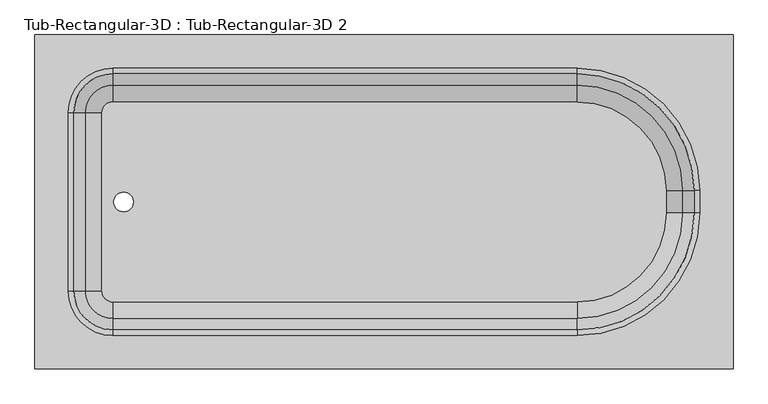
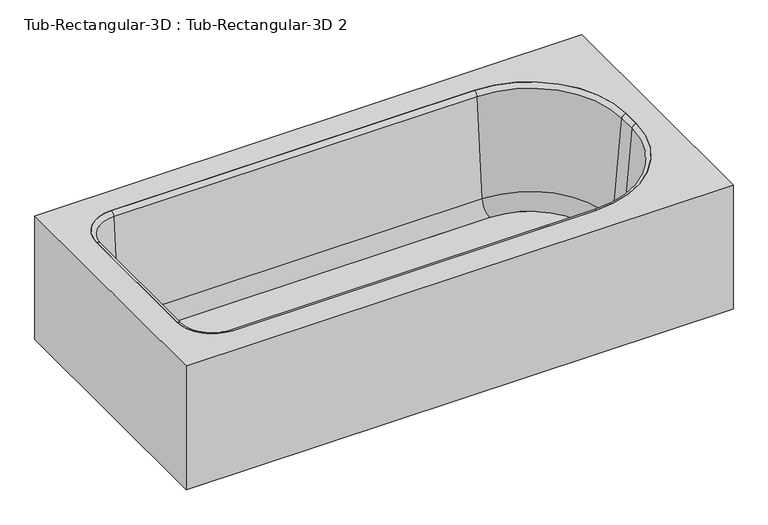
"""IFC4 building model written with IfcOpenShell, lengths in millimetres: flow terminal geometry, Tub-Rectangular-3D : Tub-Rectangular-3D 2."""

from ifc_helpers import new_model, si_unit, point, frame, frame_2d, origin, place, context, project, spatial, polyline, circle_curve, ellipse_curve, trimmed, segment, composite_curve, outline, extrude, source, transform, mapped, element, save
from ifc_brep_helpers import plane_surface, cylinder_surface, revolved_surface, advanced_brep


def tub_rectangular_3d_tub_rectangular_3d_2_a7e7f6cb(model_context):
    return source(origin(), model_context, "Body", "SolidModel", [
        advanced_brep(
        [(480.0720313, 822.325, 381.0), (-1110.6029687, 822.325, 381.0), (-1110.6029687, 60.325, 381.0), (480.0720313, 60.325, 381.0), (-932.8029687, 746.125, 381.0), (124.4720313, 746.125, 381.0), (403.8720313, 466.725, 381.0), (403.8720313, 415.925, 381.0), (124.4720313, 136.525, 381.0), (-932.8029687, 136.525, 381.0), (-1034.4029687, 238.125, 381.0), (-1034.4029687, 644.525, 381.0), (461.0220313, 803.275, 361.95), (461.0220313, 79.375, 361.95), (-1091.5529687, 79.375, 361.95), (-1091.5529687, 803.275, 361.95), (-932.8029687, 746.125, 361.95), (-1034.4029687, 644.525, 361.95), (-1034.4029687, 238.125, 361.95), (-932.8029687, 136.525, 361.95), (124.4720313, 136.525, 361.95), (403.8720313, 415.925, 361.95), (403.8720313, 466.725, 361.95), (124.4720313, 746.125, 361.95), (480.0720313, 822.325, 0.0), (-1110.6029687, 822.325, 0.0), (-1110.6029687, 60.325, 0.0), (480.0720313, 60.325, 0.0), (461.0220313, 803.275, 0.0), (-1091.5529687, 803.275, 0.0), (-1091.5529687, 79.375, 0.0), (461.0220313, 79.375, 0.0)],
        [
            (0, 1),
            (1, 2),
            (2, 3),
            (3, 0),
            (4, 5),
            (5, 6, circle_curve(frame((124.4720313, 466.725, 381.0), z_axis=(0.0, 0.0, -1.0), x_axis=(0.0, 1.0, 0.0)), 279.4)),
            (6, 7),
            (7, 8, circle_curve(frame((124.4720313, 415.925, 381.0), z_axis=(0.0, 0.0, -1.0), x_axis=(0.0, 1.0, 0.0)), 279.4)),
            (8, 9),
            (9, 10, circle_curve(frame((-932.8029687, 238.125, 381.0), z_axis=(0.0, 0.0, -1.0), x_axis=(0.0, 1.0, 0.0)), 101.6)),
            (10, 11),
            (11, 4, circle_curve(frame((-932.8029687, 644.525, 381.0), z_axis=(0.0, 0.0, -1.0), x_axis=(0.0, 1.0, 0.0)), 101.6)),
            (12, 13),
            (13, 14),
            (14, 15),
            (15, 12),
            (16, 17, circle_curve(frame((-932.8029687, 644.525, 361.95), z_axis=(0.0, 0.0, 1.0), x_axis=(0.0, 1.0, 0.0)), 101.6)),
            (17, 18),
            (18, 19, circle_curve(frame((-932.8029687, 238.125, 361.95), z_axis=(0.0, 0.0, 1.0), x_axis=(0.0, 1.0, 0.0)), 101.6)),
            (19, 20),
            (20, 21, circle_curve(frame((124.4720313, 415.925, 361.95), z_axis=(0.0, 0.0, 1.0), x_axis=(0.0, 1.0, 0.0)), 279.4)),
            (21, 22),
            (22, 23, circle_curve(frame((124.4720313, 466.725, 361.95), z_axis=(0.0, 0.0, 1.0), x_axis=(0.0, 1.0, 0.0)), 279.4)),
            (23, 16),
            (0, 24),
            (24, 25),
            (25, 1),
            (25, 26),
            (26, 2),
            (26, 27),
            (27, 3),
            (27, 24),
            (4, 16),
            (23, 5),
            (22, 6),
            (21, 7),
            (20, 8),
            (19, 9),
            (18, 10),
            (17, 11),
            (28, 29),
            (29, 30),
            (30, 31),
            (31, 28),
            (31, 13),
            (12, 28),
            (30, 14),
            (29, 15),
        ],
        [
            plane_surface(frame((-1110.6029687, 822.325, 381.0), z_axis=(0.0, 0.0, 1.0), x_axis=(-1.0, 0.0, 0.0))),
            plane_surface(frame((-1110.6029687, 822.325, 361.95), z_axis=(0.0, 0.0, -1.0), x_axis=(1.0, 0.0, 0.0))),
            plane_surface(frame((480.0720313, 822.325, 381.0), z_axis=(0.0, 1.0, 0.0), x_axis=(0.0, 0.0, -1.0))),
            plane_surface(frame((-1110.6029687, 822.325, 381.0), z_axis=(-1.0, 0.0, 0.0), x_axis=(0.0, 0.0, -1.0))),
            plane_surface(frame((-1110.6029687, 60.325, 381.0), z_axis=(0.0, -1.0, 0.0), x_axis=(0.0, 0.0, -1.0))),
            plane_surface(frame((480.0720313, 60.325, 381.0), z_axis=(1.0, 0.0, 0.0), x_axis=(0.0, 0.0, -1.0))),
            plane_surface(frame((-932.8029687, 746.125, 381.0), z_axis=(0.0, -1.0, 0.0), x_axis=(0.0, 0.0, -1.0))),
            revolved_surface(polyline([(124.4720313, 746.125, 361.95), (124.4720313, 746.125, 381.0)]), (124.4720313, 466.725, 381.0), (0.0, 0.0, -1.0)),
            plane_surface(frame((403.8720313, 466.725, 381.0), z_axis=(-1.0, 0.0, 0.0), x_axis=(0.0, 0.0, -1.0))),
            revolved_surface(polyline([(124.4720313, 695.325, 361.95), (124.4720313, 695.325, 381.0)]), (124.4720313, 415.925, 381.0), (0.0, 0.0, -1.0)),
            plane_surface(frame((124.4720313, 136.525, 381.0), z_axis=(0.0, 1.0, 0.0), x_axis=(0.0, 0.0, -1.0))),
            revolved_surface(polyline([(-932.8029687, 339.725, 361.95), (-932.8029687, 339.725, 381.0)]), (-932.8029687, 238.125, 381.0), (0.0, 0.0, -1.0)),
            plane_surface(frame((-1034.4029687, 238.125, 381.0), z_axis=(1.0, 0.0, 0.0), x_axis=(0.0, 0.0, -1.0))),
            revolved_surface(polyline([(-932.8029687, 746.125, 361.95), (-932.8029687, 746.125, 381.0)]), (-932.8029687, 644.525, 381.0), (0.0, 0.0, -1.0)),
            plane_surface(frame((-1110.6029687, 822.325, 0.0), z_axis=(0.0, 0.0, -1.0), x_axis=(1.0, 0.0, 0.0))),
            plane_surface(frame((461.0220313, 803.275, 361.95), z_axis=(-1.0, 0.0, 0.0), x_axis=(0.0, 0.0, -1.0))),
            plane_surface(frame((461.0220313, 79.375, 361.95), z_axis=(0.0, 1.0, 0.0), x_axis=(0.0, 0.0, -1.0))),
            plane_surface(frame((-1091.5529687, 79.375, 361.95), z_axis=(1.0, 0.0, 0.0), x_axis=(0.0, 0.0, -1.0))),
            plane_surface(frame((-1091.5529687, 803.275, 361.95), z_axis=(0.0, -1.0, 0.0), x_axis=(0.0, 0.0, -1.0))),
        ],
        [
            (0, [[1, 2, 3, 4], [5, 6, 7, 8, 9, 10, 11, 12]]),
            (1, [[13, 14, 15, 16], [17, 18, 19, 20, 21, 22, 23, 24]]),
            (2, [[-1, 25, 26, 27]]),
            (3, [[-2, -27, 28, 29]]),
            (4, [[-3, -29, 30, 31]]),
            (5, [[-25, -4, -31, 32]]),
            (6, [[-5, 33, -24, 34]]),
            (7, [[-6, -34, -23, 35]]),
            (8, [[-7, -35, -22, 36]]),
            (9, [[-8, -36, -21, 37]]),
            (10, [[-9, -37, -20, 38]]),
            (11, [[-10, -38, -19, 39]]),
            (12, [[-11, -39, -18, 40]]),
            (13, [[-12, -40, -17, -33]]),
            (14, [[-32, -30, -28, -26], [41, 42, 43, 44]]),
            (15, [[-44, 45, -13, 46]]),
            (16, [[-43, 47, -14, -45]]),
            (17, [[-42, 48, -15, -47]]),
            (18, [[-41, -46, -16, -48]]),
        ],
    ),
        extrude(outline(composite_curve([segment(trimmed(circle_curve(frame_2d((124.4720313, 466.725)), 202.7964741), [point((124.4720313, 669.5214741))], [point((327.2685054, 466.725))], False, "CARTESIAN"), True, "CONTINUOUS"), segment(polyline([(327.2685054, 466.725), (327.2685054, 415.925)]), True, "CONTINUOUS"), segment(trimmed(circle_curve(frame_2d((124.4720313, 415.925)), 202.7964741), [point((327.2685054, 415.925))], [point((124.4720313, 213.1285259))], False, "CARTESIAN"), True, "CONTINUOUS"), segment(polyline([(124.4720313, 213.1285259), (-932.8029687, 213.1285259)]), True, "CONTINUOUS"), segment(trimmed(circle_curve(frame_2d((-932.8029687, 238.125)), 24.9964741), [point((-932.8029687, 213.1285259))], [point((-957.7994428, 238.125))], False, "CARTESIAN"), True, "CONTINUOUS"), segment(polyline([(-957.7994428, 238.125), (-957.7994428, 644.525)]), True, "CONTINUOUS"), segment(trimmed(circle_curve(frame_2d((-932.8029687, 644.525)), 24.9964741), [point((-957.7994428, 644.525))], [point((-932.8029687, 669.5214741))], False, "CARTESIAN"), True, "CONTINUOUS"), segment(polyline([(-932.8029687, 669.5214741), (124.4720313, 669.5214741)]), True, "CONTINUOUS")], self_intersect=False), holes=[composite_curve([segment(trimmed(circle_curve(frame_2d((-908.510206, 441.325)), 22.225), [point((-908.510206, 463.55))], [point((-908.510206, 419.1))], True, "CARTESIAN"), True, "CONTINUOUS"), segment(trimmed(circle_curve(frame_2d((-908.510206, 441.325)), 22.225), [point((-908.510206, 419.1))], [point((-908.510206, 463.55))], True, "CARTESIAN"), True, "CONTINUOUS")], self_intersect=False)]), frame((0.0, 0.0, 16.863573), z_axis=(0.0, 0.0, 1.0), x_axis=(1.0, 0.0, 0.0)), (0.0, 0.0, 1.0), 19.05),
        advanced_brep(
        [(-995.7544608, 644.525, 70.6929392), (-932.8029687, 707.4764921, 70.6929392), (-932.8029687, 733.6470035, 369.8232535), (-1021.9249722, 644.525, 369.8232535), (-957.7994428, 644.525, 35.913573), (-932.8029687, 669.5214741, 35.913573), (-957.7994428, 644.525, 16.863573), (-932.8029687, 669.5214741, 16.863573), (-1034.4029687, 644.525, 16.863573), (-932.8029687, 746.125, 16.863573), (-1034.4029687, 644.525, 381.0), (-932.8029687, 746.125, 381.0), (-1021.9249722, 238.125, 369.8232535), (-995.7544608, 238.125, 70.6929392), (-957.7994428, 238.125, 35.913573), (-957.7994428, 238.125, 16.863573), (-1034.4029687, 238.125, 16.863573), (-1034.4029687, 238.125, 381.0), (-932.8029687, 175.1735079, 70.6929392), (-932.8029687, 149.0029965, 369.8232535), (-932.8029687, 213.1285259, 35.913573), (-932.8029687, 213.1285259, 16.863573), (-932.8029687, 136.525, 16.863573), (-932.8029687, 136.525, 381.0), (124.4720313, 149.0029965, 369.8232535), (124.4720313, 175.1735079, 70.6929392), (124.4720313, 213.1285259, 35.913573), (124.4720313, 213.1285259, 16.863573), (124.4720313, 136.525, 16.863573), (124.4720313, 136.525, 381.0), (365.2235234, 415.925, 70.6929392), (391.3940348, 415.925, 369.8232535), (327.2685054, 415.925, 35.913573), (327.2685054, 415.925, 16.863573), (403.8720313, 415.925, 16.863573), (403.8720313, 415.925, 381.0), (391.3940348, 466.725, 369.8232535), (365.2235234, 466.725, 70.6929392), (327.2685054, 466.725, 35.913573), (327.2685054, 466.725, 16.863573), (403.8720313, 466.725, 16.863573), (403.8720313, 466.725, 381.0), (124.4720313, 707.4764921, 70.6929392), (124.4720313, 733.6470035, 369.8232535), (124.4720313, 669.5214741, 35.913573), (124.4720313, 669.5214741, 16.863573), (124.4720313, 746.125, 16.863573), (124.4720313, 746.125, 381.0)],
        [
            (0, 1, circle_curve(frame((-932.8029687, 644.525, 70.6929392), z_axis=(0.0, 0.0, -1.0), x_axis=(0.0, 1.0, 0.0)), 62.9514921)),
            (1, 2),
            (2, 3, circle_curve(frame((-932.8029687, 644.525, 369.8232535), z_axis=(0.0, 0.0, 1.0), x_axis=(0.0, 1.0, 0.0)), 89.1220035)),
            (3, 0),
            (4, 5, circle_curve(frame((-932.8029687, 644.525, 35.913573), z_axis=(0.0, 0.0, -1.0), x_axis=(0.0, 1.0, 0.0)), 24.9964741)),
            (5, 1, circle_curve(frame((-932.8029687, 669.5214741, 74.013573), z_axis=(1.0, 0.0, 0.0), x_axis=(0.0, -1.0, 0.0)), 38.1)),
            (0, 4, circle_curve(frame((-957.7994428, 644.525, 74.013573), z_axis=(0.0, -1.0, 0.0), x_axis=(1.0, 0.0, 0.0)), 38.1)),
            (6, 7, circle_curve(frame((-932.8029687, 644.525, 16.863573), z_axis=(0.0, 0.0, -1.0), x_axis=(0.0, 1.0, 0.0)), 24.9964741)),
            (7, 5),
            (4, 6),
            (8, 9, circle_curve(frame((-932.8029687, 644.525, 16.863573), z_axis=(0.0, 0.0, -1.0), x_axis=(0.0, 1.0, 0.0)), 101.6)),
            (9, 7),
            (6, 8),
            (10, 11, circle_curve(frame((-932.8029687, 644.525, 381.0), z_axis=(0.0, 0.0, -1.0), x_axis=(0.0, 1.0, 0.0)), 101.6)),
            (11, 9),
            (8, 10),
            (2, 11, circle_curve(frame((-932.8029687, 746.125, 368.4462547), z_axis=(-1.0, 0.0, 0.0), x_axis=(0.0, -1.0, 0.0)), 12.5537453)),
            (10, 3, circle_curve(frame((-1034.4029687, 644.525, 368.4462547), z_axis=(0.0, 1.0, 0.0), x_axis=(1.0, 0.0, 0.0)), 12.5537453)),
            (3, 12),
            (12, 13),
            (13, 0),
            (13, 14, circle_curve(frame((-957.7994428, 238.125, 74.013573), z_axis=(0.0, -1.0, 0.0), x_axis=(1.0, 0.0, 0.0)), 38.1)),
            (14, 4),
            (14, 15),
            (15, 6),
            (15, 16),
            (16, 8),
            (16, 17),
            (17, 10),
            (17, 12, circle_curve(frame((-1034.4029687, 238.125, 368.4462547), z_axis=(0.0, 1.0, 0.0), x_axis=(1.0, 0.0, 0.0)), 12.5537453)),
            (18, 13, circle_curve(frame((-932.8029687, 238.125, 70.6929392), z_axis=(0.0, 0.0, -1.0), x_axis=(-1.0, 0.0, 0.0)), 62.9514921)),
            (12, 19, circle_curve(frame((-932.8029687, 238.125, 369.8232535), z_axis=(0.0, 0.0, 1.0), x_axis=(-1.0, 0.0, 0.0)), 89.1220035)),
            (19, 18),
            (20, 14, circle_curve(frame((-932.8029687, 238.125, 35.913573), z_axis=(0.0, 0.0, -1.0), x_axis=(-1.0, 0.0, 0.0)), 24.9964741)),
            (18, 20, circle_curve(frame((-932.8029687, 213.1285259, 74.013573), z_axis=(1.0, 0.0, 0.0), x_axis=(0.0, 1.0, 0.0)), 38.1)),
            (21, 15, circle_curve(frame((-932.8029687, 238.125, 16.863573), z_axis=(0.0, 0.0, -1.0), x_axis=(-1.0, 0.0, 0.0)), 24.9964741)),
            (20, 21),
            (22, 16, circle_curve(frame((-932.8029687, 238.125, 16.863573), z_axis=(0.0, 0.0, -1.0), x_axis=(-1.0, 0.0, 0.0)), 101.6)),
            (21, 22),
            (23, 17, circle_curve(frame((-932.8029687, 238.125, 381.0), z_axis=(0.0, 0.0, -1.0), x_axis=(-1.0, 0.0, 0.0)), 101.6)),
            (22, 23),
            (23, 19, circle_curve(frame((-932.8029687, 136.525, 368.4462547), z_axis=(-1.0, 0.0, 0.0), x_axis=(0.0, 1.0, 0.0)), 12.5537453)),
            (19, 24),
            (24, 25),
            (25, 18),
            (25, 26, circle_curve(frame((124.4720313, 213.1285259, 74.013573), z_axis=(1.0, 0.0, 0.0), x_axis=(0.0, 1.0, 0.0)), 38.1)),
            (26, 20),
            (26, 27),
            (27, 21),
            (27, 28),
            (28, 22),
            (28, 29),
            (29, 23),
            (29, 24, circle_curve(frame((124.4720313, 136.525, 368.4462547), z_axis=(-1.0, 0.0, 0.0), x_axis=(0.0, 1.0, 0.0)), 12.5537453)),
            (30, 25, circle_curve(frame((124.4720313, 415.925, 70.6929392), z_axis=(0.0, 0.0, -1.0), x_axis=(0.0, -1.0, 0.0)), 240.7514921)),
            (24, 31, circle_curve(frame((124.4720313, 415.925, 369.8232535), z_axis=(0.0, 0.0, 1.0), x_axis=(0.0, -1.0, 0.0)), 266.9220035)),
            (31, 30),
            (32, 26, circle_curve(frame((124.4720313, 415.925, 35.913573), z_axis=(0.0, 0.0, -1.0), x_axis=(0.0, -1.0, 0.0)), 202.7964741)),
            (30, 32, circle_curve(frame((327.2685054, 415.925, 74.013573), z_axis=(0.0, 1.0, 0.0), x_axis=(-1.0, 0.0, 0.0)), 38.1)),
            (33, 27, circle_curve(frame((124.4720313, 415.925, 16.863573), z_axis=(0.0, 0.0, -1.0), x_axis=(0.0, -1.0, 0.0)), 202.7964741)),
            (32, 33),
            (34, 28, circle_curve(frame((124.4720313, 415.925, 16.863573), z_axis=(0.0, 0.0, -1.0), x_axis=(0.0, -1.0, 0.0)), 279.4)),
            (33, 34),
            (35, 29, circle_curve(frame((124.4720313, 415.925, 381.0), z_axis=(0.0, 0.0, -1.0), x_axis=(0.0, -1.0, 0.0)), 279.4)),
            (34, 35),
            (35, 31, circle_curve(frame((403.8720313, 415.925, 368.4462547), z_axis=(0.0, -1.0, 0.0), x_axis=(-1.0, 0.0, 0.0)), 12.5537453)),
            (31, 36),
            (36, 37),
            (37, 30),
            (37, 38, circle_curve(frame((327.2685054, 466.725, 74.013573), z_axis=(0.0, 1.0, 0.0), x_axis=(-1.0, 0.0, 0.0)), 38.1)),
            (38, 32),
            (38, 39),
            (39, 33),
            (39, 40),
            (40, 34),
            (40, 41),
            (41, 35),
            (41, 36, circle_curve(frame((403.8720313, 466.725, 368.4462547), z_axis=(0.0, -1.0, 0.0), x_axis=(-1.0, 0.0, 0.0)), 12.5537453)),
            (42, 37, circle_curve(frame((124.4720313, 466.725, 70.6929392), z_axis=(0.0, 0.0, -1.0), x_axis=(1.0, 0.0, 0.0)), 240.7514921)),
            (36, 43, circle_curve(frame((124.4720313, 466.725, 369.8232535), z_axis=(0.0, 0.0, 1.0), x_axis=(1.0, 0.0, 0.0)), 266.9220035)),
            (43, 42),
            (44, 38, circle_curve(frame((124.4720313, 466.725, 35.913573), z_axis=(0.0, 0.0, -1.0), x_axis=(1.0, 0.0, 0.0)), 202.7964741)),
            (42, 44, circle_curve(frame((124.4720313, 669.5214741, 74.013573), z_axis=(-1.0, 0.0, 0.0), x_axis=(0.0, -1.0, 0.0)), 38.1)),
            (45, 39, circle_curve(frame((124.4720313, 466.725, 16.863573), z_axis=(0.0, 0.0, -1.0), x_axis=(1.0, 0.0, 0.0)), 202.7964741)),
            (44, 45),
            (46, 40, circle_curve(frame((124.4720313, 466.725, 16.863573), z_axis=(0.0, 0.0, -1.0), x_axis=(1.0, 0.0, 0.0)), 279.4)),
            (45, 46),
            (47, 41, circle_curve(frame((124.4720313, 466.725, 381.0), z_axis=(0.0, 0.0, -1.0), x_axis=(1.0, 0.0, 0.0)), 279.4)),
            (46, 47),
            (47, 43, circle_curve(frame((124.4720313, 746.125, 368.4462547), z_axis=(1.0, 0.0, 0.0), x_axis=(0.0, -1.0, 0.0)), 12.5537453)),
            (43, 2),
            (1, 42),
            (5, 44),
            (7, 45),
            (9, 46),
            (11, 47),
        ],
        [
            revolved_surface(polyline([(-932.8029687, 733.6470035, 369.8232535), (-932.8029687, 707.4764921, 70.6929392)]), (-932.8029687, 644.525, 381.0), (0.0, 0.0, 1.0)),
            revolved_surface(trimmed(ellipse_curve(frame((-932.8029687, 669.5214741, 74.013573), z_axis=(-1.0, 0.0, 0.0), x_axis=(0.0, -1.0, 0.0)), 38.1, 38.1), [point((-932.8029687, 707.4764921, 70.6929392))], [point((-932.8029687, 669.5214741, 35.913573))], True, "CARTESIAN"), (-932.8029687, 644.525, 381.0), (0.0, 0.0, 1.0)),
            revolved_surface(polyline([(-932.8029687, 669.5214741, 35.913572999999985), (-932.8029687, 669.5214741, 16.863572999999974)]), (-932.8029687, 644.525, 381.0), (0.0, 0.0, 1.0)),
            plane_surface(frame((-932.8029687, 644.525, 16.863573), z_axis=(0.0, 0.0, -1.0), x_axis=(0.0, 1.0, 0.0))),
            cylinder_surface(frame((-932.8029687, 644.525, 381.0), z_axis=(0.0, 0.0, 1.0), x_axis=(0.0, 1.0, 0.0)), 101.6),
            revolved_surface(trimmed(ellipse_curve(frame((-932.8029687, 746.125, 368.4462547), z_axis=(1.0, 0.0, 0.0), x_axis=(0.0, -1.0, 0.0)), 12.5537453, 12.5537453), [point((-932.8029687, 746.125, 381.0))], [point((-932.8029687, 733.6470035, 369.8232535))], True, "CARTESIAN"), (-932.8029687, 644.525, 381.0), (0.0, 0.0, 1.0)),
            plane_surface(frame((-1021.9249722, 644.525, 369.8232535), z_axis=(0.9961946980917458, 0.0, 0.08715574274765595), x_axis=(0.0, -1.0, 0.0))),
            revolved_surface(polyline([(-919.6994427999999, 238.125, 74.013573), (-919.6994427999999, 644.525, 74.013573)]), (-957.7994428, 644.525, 74.013573), (0.0, -1.0, 0.0)),
            plane_surface(frame((-957.7994428, 644.525, 35.913573), z_axis=(1.0, 0.0, 0.0), x_axis=(0.0, -1.0, 0.0))),
            plane_surface(frame((-957.7994428, 644.525, 16.863573), z_axis=(0.0, 0.0, -1.0), x_axis=(0.0, -1.0, 0.0))),
            plane_surface(frame((-1034.4029687, 644.525, 16.863573), z_axis=(-1.0, 0.0, 0.0), x_axis=(0.0, -1.0, 0.0))),
            cylinder_surface(frame((-1034.4029687, 644.525, 368.4462547), z_axis=(0.0, 1.0, 0.0), x_axis=(1.0, 0.0, 0.0)), 12.5537453),
            revolved_surface(polyline([(-1021.9249722, 238.125, 369.8232535), (-995.7544608, 238.125, 70.6929392)]), (-932.8029687, 238.125, 381.0), (0.0, 0.0, 1.0)),
            revolved_surface(trimmed(ellipse_curve(frame((-957.7994428, 238.125, 74.013573), z_axis=(0.0, -1.0, 0.0), x_axis=(1.0, 0.0, 0.0)), 38.1, 38.1), [point((-995.7544608, 238.125, 70.6929392))], [point((-957.7994428, 238.125, 35.913573))], True, "CARTESIAN"), (-932.8029687, 238.125, 381.0), (0.0, 0.0, 1.0)),
            revolved_surface(polyline([(-957.7994428, 238.125, 35.913572999999985), (-957.7994428, 238.125, 16.863572999999974)]), (-932.8029687, 238.125, 381.0), (0.0, 0.0, 1.0)),
            plane_surface(frame((-932.8029687, 238.125, 16.863573), z_axis=(0.0, 0.0, -1.0), x_axis=(-1.0, 0.0, 0.0))),
            cylinder_surface(frame((-932.8029687, 238.125, 381.0), z_axis=(0.0, 0.0, 1.0), x_axis=(-1.0, 0.0, 0.0)), 101.6),
            revolved_surface(trimmed(ellipse_curve(frame((-1034.4029687, 238.125, 368.4462547), z_axis=(0.0, 1.0, 0.0), x_axis=(1.0, 0.0, 0.0)), 12.5537453, 12.5537453), [point((-1034.4029687, 238.125, 381.0))], [point((-1021.9249722, 238.125, 369.8232535))], True, "CARTESIAN"), (-932.8029687, 238.125, 381.0), (0.0, 0.0, 1.0)),
            plane_surface(frame((-932.8029687, 149.0029965, 369.8232535), z_axis=(0.0, 0.9961946980917461, 0.08715574274765271), x_axis=(1.0, 0.0, 0.0))),
            revolved_surface(polyline([(124.47203129999991, 251.2285259, 74.013573), (-932.8029687, 251.2285259, 74.013573)]), (-932.8029687, 213.1285259, 74.013573), (1.0, 0.0, 0.0)),
            plane_surface(frame((-932.8029687, 213.1285259, 35.913573), z_axis=(0.0, 1.0, 0.0), x_axis=(1.0, 0.0, 0.0))),
            plane_surface(frame((-932.8029687, 213.1285259, 16.863573), z_axis=(0.0, 0.0, -1.0), x_axis=(1.0, 0.0, 0.0))),
            plane_surface(frame((-932.8029687, 136.525, 16.863573), z_axis=(0.0, -1.0, 0.0), x_axis=(1.0, 0.0, 0.0))),
            cylinder_surface(frame((-932.8029687, 136.525, 368.4462547), z_axis=(-1.0, 0.0, 0.0), x_axis=(0.0, 1.0, 0.0)), 12.5537453),
            revolved_surface(polyline([(124.4720313, 149.0029965, 369.8232535), (124.4720313, 175.1735079, 70.6929392)]), (124.4720313, 415.925, 381.0), (0.0, 0.0, 1.0)),
            revolved_surface(trimmed(ellipse_curve(frame((124.4720313, 213.1285259, 74.013573), z_axis=(1.0, 0.0, 0.0), x_axis=(0.0, 1.0, 0.0)), 38.1, 38.1), [point((124.4720313, 175.1735079, 70.6929392))], [point((124.4720313, 213.1285259, 35.913573))], True, "CARTESIAN"), (124.4720313, 415.925, 381.0), (0.0, 0.0, 1.0)),
            revolved_surface(polyline([(124.4720313, 213.1285259, 35.913572999999985), (124.4720313, 213.1285259, 16.863572999999974)]), (124.4720313, 415.925, 381.0), (0.0, 0.0, 1.0)),
            plane_surface(frame((124.4720313, 415.925, 16.863573), z_axis=(0.0, 0.0, -1.0), x_axis=(0.0, -1.0, 0.0))),
            cylinder_surface(frame((124.4720313, 415.925, 381.0), z_axis=(0.0, 0.0, 1.0), x_axis=(0.0, -1.0, 0.0)), 279.4),
            revolved_surface(trimmed(ellipse_curve(frame((124.4720313, 136.525, 368.4462547), z_axis=(-1.0, 0.0, 0.0), x_axis=(0.0, 1.0, 0.0)), 12.5537453, 12.5537453), [point((124.4720313, 136.525, 381.0))], [point((124.4720313, 149.0029965, 369.8232535))], True, "CARTESIAN"), (124.4720313, 415.925, 381.0), (0.0, 0.0, 1.0)),
            plane_surface(frame((391.3940348, 415.925, 369.8232535), z_axis=(-0.9961946980917464, 0.0, 0.08715574274764948), x_axis=(0.0, 1.0, 0.0))),
            revolved_surface(polyline([(289.16850539999996, 466.725, 74.013573), (289.16850539999996, 415.925, 74.013573)]), (327.2685054, 415.925, 74.013573), (0.0, 1.0, 0.0)),
            plane_surface(frame((327.2685054, 415.925, 35.913573), z_axis=(-1.0, 0.0, 0.0), x_axis=(0.0, 1.0, 0.0))),
            plane_surface(frame((327.2685054, 415.925, 16.863573), z_axis=(0.0, 0.0, -1.0), x_axis=(0.0, 1.0, 0.0))),
            plane_surface(frame((403.8720313, 415.925, 16.863573), z_axis=(1.0, 0.0, 0.0), x_axis=(0.0, 1.0, 0.0))),
            cylinder_surface(frame((403.8720313, 415.925, 368.4462547), z_axis=(0.0, -1.0, 0.0), x_axis=(-1.0, 0.0, 0.0)), 12.5537453),
            revolved_surface(polyline([(391.3940348, 466.725, 369.8232535), (365.2235234, 466.725, 70.6929392)]), (124.4720313, 466.725, 381.0), (0.0, 0.0, 1.0)),
            revolved_surface(trimmed(ellipse_curve(frame((327.2685054, 466.725, 74.013573), z_axis=(0.0, 1.0, 0.0), x_axis=(-1.0, 0.0, 0.0)), 38.1, 38.1), [point((365.2235234, 466.725, 70.6929392))], [point((327.2685054, 466.725, 35.913573))], True, "CARTESIAN"), (124.4720313, 466.725, 381.0), (0.0, 0.0, 1.0)),
            revolved_surface(polyline([(327.2685054, 466.725, 35.913572999999985), (327.2685054, 466.725, 16.863572999999974)]), (124.4720313, 466.725, 381.0), (0.0, 0.0, 1.0)),
            plane_surface(frame((124.4720313, 466.725, 16.863573), z_axis=(0.0, 0.0, -1.0), x_axis=(1.0, 0.0, 0.0))),
            cylinder_surface(frame((124.4720313, 466.725, 381.0), z_axis=(0.0, 0.0, 1.0), x_axis=(1.0, 0.0, 0.0)), 279.4),
            revolved_surface(trimmed(ellipse_curve(frame((403.8720313, 466.725, 368.4462547), z_axis=(0.0, -1.0, 0.0), x_axis=(-1.0, 0.0, 0.0)), 12.5537453, 12.5537453), [point((403.8720313, 466.725, 381.0))], [point((391.3940348, 466.725, 369.8232535))], True, "CARTESIAN"), (124.4720313, 466.725, 381.0), (0.0, 0.0, 1.0)),
            plane_surface(frame((124.4720313, 733.6470035, 369.8232535), z_axis=(0.0, -0.9961946980917461, 0.08715574274765271), x_axis=(-1.0, 0.0, 0.0))),
            revolved_surface(polyline([(-932.8029686999998, 631.4214741, 74.013573), (124.4720313, 631.4214741, 74.013573)]), (124.4720313, 669.5214741, 74.013573), (-1.0, 0.0, 0.0)),
            plane_surface(frame((124.4720313, 669.5214741, 35.913573), z_axis=(0.0, -1.0, 0.0), x_axis=(-1.0, 0.0, 0.0))),
            plane_surface(frame((124.4720313, 669.5214741, 16.863573), z_axis=(0.0, 0.0, -1.0), x_axis=(-1.0, 0.0, 0.0))),
            plane_surface(frame((124.4720313, 746.125, 16.863573), z_axis=(0.0, 1.0, 0.0), x_axis=(-1.0, 0.0, 0.0))),
            cylinder_surface(frame((124.4720313, 746.125, 368.4462547), z_axis=(1.0, 0.0, 0.0), x_axis=(0.0, -1.0, 0.0)), 12.5537453),
        ],
        [
            (0, [[1, 2, 3, 4]]),
            (1, [[5, 6, -1, 7]]),
            (2, [[8, 9, -5, 10]]),
            (3, [[11, 12, -8, 13]]),
            (4, [[14, 15, -11, 16]]),
            (5, [[-3, 17, -14, 18]]),
            (6, [[-4, 19, 20, 21]]),
            (7, [[-7, -21, 22, 23]]),
            (8, [[-10, -23, 24, 25]]),
            (9, [[-13, -25, 26, 27]]),
            (10, [[-16, -27, 28, 29]]),
            (11, [[-18, -29, 30, -19]]),
            (12, [[31, -20, 32, 33]]),
            (13, [[34, -22, -31, 35]]),
            (14, [[36, -24, -34, 37]]),
            (15, [[38, -26, -36, 39]]),
            (16, [[40, -28, -38, 41]]),
            (17, [[-32, -30, -40, 42]]),
            (18, [[-33, 43, 44, 45]]),
            (19, [[-35, -45, 46, 47]]),
            (20, [[-37, -47, 48, 49]]),
            (21, [[-39, -49, 50, 51]]),
            (22, [[-41, -51, 52, 53]]),
            (23, [[-42, -53, 54, -43]]),
            (24, [[55, -44, 56, 57]]),
            (25, [[58, -46, -55, 59]]),
            (26, [[60, -48, -58, 61]]),
            (27, [[62, -50, -60, 63]]),
            (28, [[64, -52, -62, 65]]),
            (29, [[-56, -54, -64, 66]]),
            (30, [[-57, 67, 68, 69]]),
            (31, [[-59, -69, 70, 71]]),
            (32, [[-61, -71, 72, 73]]),
            (33, [[-63, -73, 74, 75]]),
            (34, [[-65, -75, 76, 77]]),
            (35, [[-66, -77, 78, -67]]),
            (36, [[79, -68, 80, 81]]),
            (37, [[82, -70, -79, 83]]),
            (38, [[84, -72, -82, 85]]),
            (39, [[86, -74, -84, 87]]),
            (40, [[88, -76, -86, 89]]),
            (41, [[-80, -78, -88, 90]]),
            (42, [[-81, 91, -2, 92]]),
            (43, [[-83, -92, -6, 93]]),
            (44, [[-85, -93, -9, 94]]),
            (45, [[-87, -94, -12, 95]]),
            (46, [[-89, -95, -15, 96]]),
            (47, [[-90, -96, -17, -91]]),
        ],
    ),
    ])


if __name__ == "__main__":
    model = new_model("IFC4")
    model_context = context("Model", 3, world=origin())
    ifc_project = project(units=[si_unit("LENGTHUNIT", "METRE", prefix="MILLI")], contexts=[model_context])
    site = spatial("IfcSite", under=ifc_project)
    building = spatial("IfcBuilding", under=site)
    placement = place(None, origin())
    tub_rectangular_3d_tub_rectangular_3d_2_shape = tub_rectangular_3d_tub_rectangular_3d_2_a7e7f6cb(model_context)
    element("IfcFlowTerminal", 1, ObjectType="Tub-Rectangular-3D : Tub-Rectangular-3D 2", at=placement, inside=building, context=model_context, shape_type="MappedRepresentation", body=[
        mapped(tub_rectangular_3d_tub_rectangular_3d_2_shape, transform((0.0, 0.0, 0.0), x_axis=(1.0, 0.0, 0.0), y_axis=(0.0, 1.0, 0.0), z_axis=(0.0, 0.0, 1.0))),
    ])
    save(model, "model.ifc")

# Revit data of these elements
# Type "Tub-Rectangular-3D : Tub-Rectangular-3D 2"
#   Assembly Code = "D2010500"
#   Depth = 2' - 6"
#   Height = 1' - 3"
#   Width = 5' - 2 5/8"
#   Tub Material = Porcelain, Ivory
# Element 1 (IfcFlowTerminal, "Tub-Rectangular-3D : Tub-Rectangular-3D 2")
#   Materials on its faces: "Porcelain, Ivory"
# Materials
#   "Porcelain, Ivory": class "Ceramic", colour RGB 247 247 239, transparency 0, Description = "Porcelain, ivory", Cost = 0
